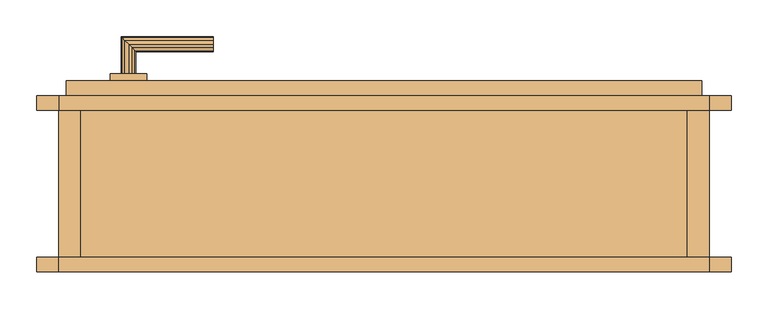
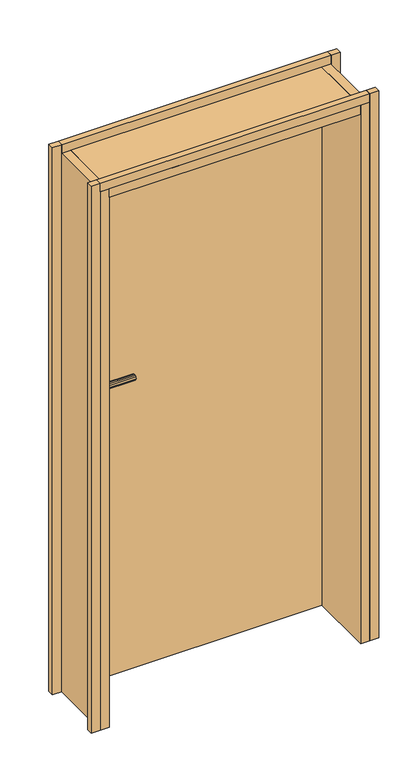
"""IFC4 building model written with IfcOpenShell, lengths in millimetres: door geometry, Tür."""

from ifc_helpers import new_model, si_unit, frame, origin, place, context, project, spatial, polyline, outline, extrude, faceted_brep, source, transform, mapped, element, save


def door_a0d39162(model_context):
    return source(origin(), model_context, "Body", "SolidModel", [
        extrude(outline(polyline([(885.0, -20.0), (855.0, -20.0), (855.0, 220.0), (885.0, 220.0), (885.0, -20.0)])), frame((0.0, 0.0, 140.0), z_axis=(0.0, 0.0, 1.0), x_axis=(1.0, 0.0, 0.0)), (0.0, 0.0, 1.0), 1870.0),
        extrude(outline(polyline([(0.0, 200.0), (-30.0, 200.0), (-30.0, 220.0), (0.0, 220.0), (0.0, 200.0)])), frame((0.0, 0.0, 140.0), z_axis=(0.0, 0.0, 1.0), x_axis=(1.0, 0.0, 0.0)), (0.0, 0.0, 1.0), 1900.0),
        extrude(outline(polyline([(855.0, -20.0), (30.0, -20.0), (30.0, 220.0), (855.0, 220.0), (855.0, -20.0)])), frame((0.0, 0.0, 1980.0), z_axis=(0.0, 0.0, 1.0), x_axis=(1.0, 0.0, 0.0)), (0.0, 0.0, 1.0), 30.0),
        extrude(outline(polyline([(885.0, -20.0), (0.0, -20.0), (0.0, 0.0), (885.0, 0.0), (885.0, -20.0)])), frame((0.0, 0.0, 2010.0), z_axis=(0.0, 0.0, 1.0), x_axis=(1.0, 0.0, 0.0)), (0.0, 0.0, 1.0), 30.0),
        extrude(outline(polyline([(120.0, 240.0), (70.0, 240.0), (70.0, 250.0), (120.0, 250.0), (120.0, 240.0)])), frame((0.0, 0.0, 1050.0), z_axis=(0.0, 0.0, 1.0), x_axis=(1.0, 0.0, 0.0)), (0.0, 0.0, 1.0), 215.0),
        faceted_brep([(100.0, 250.0, 1198.660254), (95.0, 250.0, 1200.0), (90.0, 250.0, 1198.660254), (86.339746, 250.0, 1195.0), (85.0, 250.0, 1190.0), (86.339746, 250.0, 1185.0), (90.0, 250.0, 1181.339746), (95.0, 250.0, 1180.0), (100.0, 250.0, 1181.339746), (103.660254, 250.0, 1185.0), (105.0, 250.0, 1190.0), (103.660254, 250.0, 1195.0), (95.0, 290.0, 1200.0), (90.0, 295.0, 1198.660254), (86.339746, 298.660254, 1195.0), (85.0, 300.0, 1190.0), (86.339746, 298.660254, 1185.0), (90.0, 295.0, 1181.339746), (95.0, 290.0, 1180.0), (100.0, 285.0, 1181.339746), (103.660254, 281.339746, 1185.0), (105.0, 280.0, 1190.0), (103.660254, 281.339746, 1195.0), (100.0, 285.0, 1198.660254), (210.0, 295.0, 1198.660254), (210.0, 290.0, 1200.0), (210.0, 285.0, 1198.660254), (210.0, 281.339746, 1195.0), (210.0, 280.0, 1190.0), (210.0, 281.339746, 1185.0), (210.0, 285.0, 1181.339746), (210.0, 290.0, 1180.0), (210.0, 295.0, 1181.339746), (210.0, 298.660254, 1185.0), (210.0, 300.0, 1190.0), (210.0, 298.660254, 1195.0)], [[[0, 1, 2, 3, 4, 5, 6, 7, 8, 9, 10, 11]], [[2, 1, 12, 13]], [[3, 2, 13, 14]], [[4, 3, 14, 15]], [[5, 4, 15, 16]], [[6, 5, 16, 17]], [[7, 6, 17, 18]], [[8, 7, 18, 19]], [[9, 8, 19, 20]], [[10, 9, 20, 21]], [[11, 10, 21, 22]], [[0, 11, 22, 23]], [[1, 0, 23, 12]], [[24, 25, 26, 27, 28, 29, 30, 31, 32, 33, 34, 35]], [[13, 12, 25, 24]], [[14, 13, 24, 35]], [[15, 14, 35, 34]], [[16, 15, 34, 33]], [[17, 16, 33, 32]], [[18, 17, 32, 31]], [[19, 18, 31, 30]], [[20, 19, 30, 29]], [[21, 20, 29, 28]], [[22, 21, 28, 27]], [[23, 22, 27, 26]], [[12, 23, 26, 25]]]),
        faceted_brep([(90.0, 190.0, 1198.660254), (95.0, 190.0, 1200.0), (100.0, 190.0, 1198.660254), (103.660254, 190.0, 1195.0), (105.0, 190.0, 1190.0), (103.660254, 190.0, 1185.0), (100.0, 190.0, 1181.339746), (95.0, 190.0, 1180.0), (90.0, 190.0, 1181.339746), (86.339746, 190.0, 1185.0), (85.0, 190.0, 1190.0), (86.339746, 190.0, 1195.0), (95.0, 150.0, 1200.0), (90.0, 145.0, 1198.660254), (86.339746, 141.339746, 1195.0), (85.0, 140.0, 1190.0), (86.339746, 141.339746, 1185.0), (90.0, 145.0, 1181.339746), (95.0, 150.0, 1180.0), (100.0, 155.0, 1181.339746), (103.660254, 158.660254, 1185.0), (105.0, 160.0, 1190.0), (103.660254, 158.660254, 1195.0), (100.0, 155.0, 1198.660254), (210.0, 155.0, 1198.660254), (210.0, 150.0, 1200.0), (210.0, 145.0, 1198.660254), (210.0, 141.339746, 1195.0), (210.0, 140.0, 1190.0), (210.0, 141.339746, 1185.0), (210.0, 145.0, 1181.339746), (210.0, 150.0, 1180.0), (210.0, 155.0, 1181.339746), (210.0, 158.660254, 1185.0), (210.0, 160.0, 1190.0), (210.0, 158.660254, 1195.0)], [[[0, 1, 2, 3, 4, 5, 6, 7, 8, 9, 10, 11]], [[12, 1, 0, 13]], [[13, 0, 11, 14]], [[14, 11, 10, 15]], [[15, 10, 9, 16]], [[16, 9, 8, 17]], [[17, 8, 7, 18]], [[18, 7, 6, 19]], [[19, 6, 5, 20]], [[20, 5, 4, 21]], [[21, 4, 3, 22]], [[22, 3, 2, 23]], [[23, 2, 1, 12]], [[24, 25, 26, 27, 28, 29, 30, 31, 32, 33, 34, 35]], [[25, 12, 13, 26]], [[26, 13, 14, 27]], [[27, 14, 15, 28]], [[28, 15, 16, 29]], [[29, 16, 17, 30]], [[30, 17, 18, 31]], [[31, 18, 19, 32]], [[32, 19, 20, 33]], [[33, 20, 21, 34]], [[34, 21, 22, 35]], [[35, 22, 23, 24]], [[24, 23, 12, 25]]]),
        extrude(outline(polyline([(70.0, 190.0), (70.0, 200.0), (120.0, 200.0), (120.0, 190.0), (70.0, 190.0)])), frame((0.0, 0.0, 1050.0), z_axis=(0.0, 0.0, 1.0), x_axis=(1.0, 0.0, 0.0)), (0.0, 0.0, 1.0), 215.0),
        extrude(outline(polyline([(875.0, 200.0), (10.0, 200.0), (10.0, 240.0), (875.0, 240.0), (875.0, 200.0)])), frame((0.0, 0.0, 140.0), z_axis=(0.0, 0.0, 1.0), x_axis=(1.0, 0.0, 0.0)), (0.0, 0.0, 1.0), 1860.0),
        extrude(outline(polyline([(915.0, 0.0), (915.0, -20.0), (885.0, -20.0), (885.0, 0.0), (915.0, 0.0)])), frame((0.0, 0.0, 140.0), z_axis=(0.0, 0.0, 1.0), x_axis=(1.0, 0.0, 0.0)), (0.0, 0.0, 1.0), 1900.0),
        extrude(outline(polyline([(0.0, -20.0), (-30.0, -20.0), (-30.0, 0.0), (0.0, 0.0), (0.0, -20.0)])), frame((0.0, 0.0, 140.0), z_axis=(0.0, 0.0, 1.0), x_axis=(1.0, 0.0, 0.0)), (0.0, 0.0, 1.0), 1900.0),
        extrude(outline(polyline([(885.0, 200.0), (0.0, 200.0), (0.0, 220.0), (885.0, 220.0), (885.0, 200.0)])), frame((0.0, 0.0, 2010.0), z_axis=(0.0, 0.0, 1.0), x_axis=(1.0, 0.0, 0.0)), (0.0, 0.0, 1.0), 30.0),
        extrude(outline(polyline([(30.0, -20.0), (0.0, -20.0), (0.0, 220.0), (30.0, 220.0), (30.0, -20.0)])), frame((0.0, 0.0, 140.0), z_axis=(0.0, 0.0, 1.0), x_axis=(1.0, 0.0, 0.0)), (0.0, 0.0, 1.0), 1870.0),
        extrude(outline(polyline([(915.0, 220.0), (915.0, 200.0), (885.0, 200.0), (885.0, 220.0), (915.0, 220.0)])), frame((0.0, 0.0, 140.0), z_axis=(0.0, 0.0, 1.0), x_axis=(1.0, 0.0, 0.0)), (0.0, 0.0, 1.0), 1900.0),
    ])


if __name__ == "__main__":
    model = new_model("IFC4")
    model_context = context("Model", 3, world=origin())
    ifc_project = project(units=[si_unit("LENGTHUNIT", "METRE", prefix="MILLI")], contexts=[model_context])
    site = spatial("IfcSite", under=ifc_project)
    building = spatial("IfcBuilding", under=site)
    placement = place(None, origin())
    door_shape = door_a0d39162(model_context)
    element("IfcDoor", 1, ObjectType="Tür", at=placement, inside=building, context=model_context, shape_type="MappedRepresentation", body=[
        mapped(door_shape, transform((0.0, 0.0, 0.0), x_axis=(1.0, 0.0, 0.0), y_axis=(0.0, 1.0, 0.0), z_axis=(0.0, 0.0, 1.0))),
    ])
    save(model, "model.ifc")

# Revit data of these elements
# Type "Tür"
#   Type Mark = "35"
# Element 1 (IfcDoor, "Tür")
#   Materials on its faces: "tuer_beschlag", "tuer_holzzarge"
# Materials
#   "tuer_beschlag": class "Unassigned", colour RGB 128 128 128, transparency 0
#   "tuer_holzzarge": class "Unassigned", colour RGB 255 255 255, transparency 0
